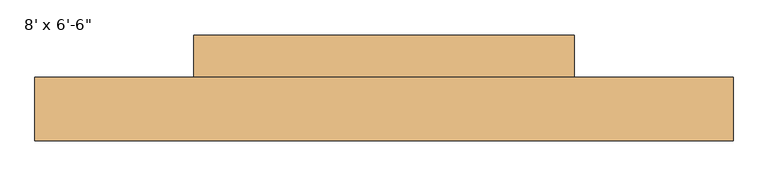
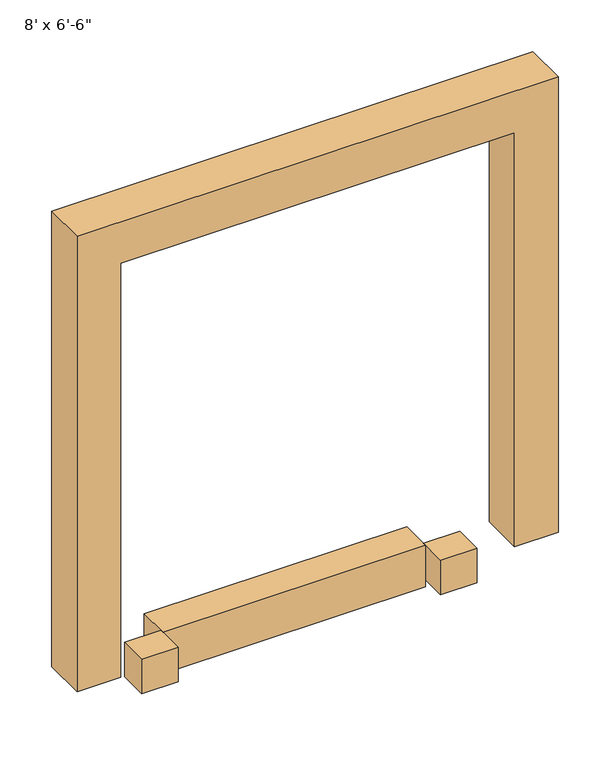
"""IFC4 building model written with IfcOpenShell, lengths in millimetres: door geometry."""

import ifcopenshell
import ifcopenshell.guid

model = None  # the IFC model being written
_history = None  # IfcOwnerHistory: only IFC2X3 demands one
_inside = {}  # id of a spatial element -> (the spatial element, [elements in it])
_under = {}  # id of a project, library or spatial element -> (it, [spatial elements below it])
_declared = {}  # id of a project -> (the project, [libraries it declares])
_typed = {}  # id of a type object -> (the type object, [elements of that type])
_made_of = {}  # id of a material, layer set ... -> (it, [elements and type objects made of it])


def new_model(schema):
    """Start an empty IFC model of exactly this schema.

    Asked for "IFC4X3", IfcOpenShell would pick the latest addendum, in which some entities
    have other attributes; the version numbers below select the first issue.
    IFC2X3 requires an IfcOwnerHistory on every rooted entity: one is made here for all.
    """
    global model, _history
    if schema == "IFC4X3":
        model = ifcopenshell.file(schema_version=(4, 3, 0, 0))
    else:
        model = ifcopenshell.file(schema=schema)
    _inside.clear()
    _under.clear()
    _declared.clear()
    _typed.clear()
    _made_of.clear()
    _history = None
    if model.schema == "IFC2X3":
        org = make("IfcOrganization", Name="unknown")
        user = make(
            "IfcPersonAndOrganization",
            ThePerson=make("IfcPerson", FamilyName="unknown"),
            TheOrganization=org,
        )
        app = make(
            "IfcApplication",
            ApplicationDeveloper=org,
            Version="unknown",
            ApplicationFullName="unknown",
            ApplicationIdentifier="unknown",
        )
        _history = make(
            "IfcOwnerHistory",
            OwningUser=user,
            OwningApplication=app,
            ChangeAction="ADDED",
            CreationDate=0,
        )
    return model


def make(cls, **values):
    """One entity of the class cls with the attributes given. An attribute that is None is left unset."""
    return model.create_entity(
        cls, **{name: value for name, value in values.items() if value is not None}
    )


def rooted(cls, **values):
    """An entity with a GlobalId (a new one), such as an element, a storey or a relation."""
    return make(cls, GlobalId=ifcopenshell.guid.new(), OwnerHistory=_history, **values)


def si_unit(unit_type, name, prefix=None):
    """IfcSIUnit, for example si_unit("LENGTHUNIT", "METRE", prefix="MILLI")."""
    return make("IfcSIUnit", UnitType=unit_type, Prefix=prefix, Name=name)


def assignment(units):
    """IfcUnitAssignment: the units of a project."""
    return None if units is None else make("IfcUnitAssignment", Units=units)


def point(xyz):
    """IfcCartesianPoint."""
    return None if xyz is None else make("IfcCartesianPoint", Coordinates=xyz)


def direction(xyz):
    """IfcDirection."""
    return None if xyz is None else make("IfcDirection", DirectionRatios=xyz)


def frame(location, z_axis=None, x_axis=None):
    """IfcAxis2Placement3D, a coordinate frame: its origin and axes. An axis left out is left unset."""
    return make(
        "IfcAxis2Placement3D",
        Location=point(location),
        Axis=direction(z_axis),
        RefDirection=direction(x_axis),
    )


def origin():
    """The frame at (0, 0, 0) with its axes left unset."""
    return frame((0.0, 0.0, 0.0))


def place(relative_to, where):
    """IfcLocalPlacement: puts the frame where relative to a parent placement (None: the world)."""
    return make(
        "IfcLocalPlacement", PlacementRelTo=relative_to, RelativePlacement=where
    )


def context(
    kind, dimensions, precision=None, world=None, true_north=None, identifier=None
):
    """IfcGeometricRepresentationContext, for example the 3D "Model" context."""
    return make(
        "IfcGeometricRepresentationContext",
        ContextIdentifier=identifier,
        ContextType=kind,
        CoordinateSpaceDimension=dimensions,
        Precision=precision,
        WorldCoordinateSystem=world,
        TrueNorth=true_north,
    )


def project(units=None, contexts=None):
    """IfcProject with its units and contexts."""
    return rooted(
        "IfcProject",
        Name="project",
        RepresentationContexts=contexts,
        UnitsInContext=assignment(units),
    )


def spatial(cls, under=None, at=None, **own):
    """A site, building, storey or space (cls), placed at a placement, below another one or the project."""
    s = rooted(cls, ObjectPlacement=at, **own)
    if under is not None:
        _under.setdefault(under.id(), (under, []))[1].append(s)
    return s


def polyline(points):
    """IfcPolyline through the points."""
    return make("IfcPolyline", Points=[point(p) for p in points])


def outline(outer, holes=None, kind="AREA"):
    """IfcArbitraryClosedProfileDef: a profile drawn as a closed curve; with holes, ...WithVoids."""
    if holes is None:
        return make("IfcArbitraryClosedProfileDef", ProfileType=kind, OuterCurve=outer)
    return make(
        "IfcArbitraryProfileDefWithVoids",
        ProfileType=kind,
        OuterCurve=outer,
        InnerCurves=holes,
    )


def extrude(swept, where, along, depth):
    """IfcExtrudedAreaSolid: the profile swept, set in the frame where, extruded along a direction by depth."""
    return make(
        "IfcExtrudedAreaSolid",
        SweptArea=swept,
        Position=where,
        ExtrudedDirection=direction(along),
        Depth=depth,
    )


def shape(context_of_items, identifier, shape_type, items):
    """IfcShapeRepresentation: the items that make up one representation, for example the "Body"."""
    return make(
        "IfcShapeRepresentation",
        ContextOfItems=context_of_items,
        RepresentationIdentifier=identifier,
        RepresentationType=shape_type,
        Items=items,
    )


def source(mapping_origin, context_of_items, identifier, shape_type, items):
    """IfcRepresentationMap: a shape defined once, which mapped items show again and again."""
    return make(
        "IfcRepresentationMap",
        MappingOrigin=mapping_origin,
        MappedRepresentation=shape(context_of_items, identifier, shape_type, items),
    )


def transform(
    local_origin,
    x_axis=None,
    y_axis=None,
    z_axis=None,
    scale=None,
    scale2=None,
    scale3=None,
    uniform=True,
):
    """IfcCartesianTransformationOperator3D, or its non-uniform kind. x_axis, y_axis, z_axis: its Axis1, 2, 3."""
    if uniform:
        return make(
            "IfcCartesianTransformationOperator3D",
            Axis1=direction(x_axis),
            Axis2=direction(y_axis),
            LocalOrigin=point(local_origin),
            Scale=scale,
            Axis3=direction(z_axis),
        )
    return make(
        "IfcCartesianTransformationOperator3DnonUniform",
        Axis1=direction(x_axis),
        Axis2=direction(y_axis),
        LocalOrigin=point(local_origin),
        Scale=scale,
        Axis3=direction(z_axis),
        Scale2=scale2,
        Scale3=scale3,
    )


def mapped(mapping_source, mapping_target):
    """IfcMappedItem: shows the shape of a source again, moved by a transform."""
    return make(
        "IfcMappedItem", MappingSource=mapping_source, MappingTarget=mapping_target
    )


def made_of(thing, what):
    """Note that an element or type object is made of a material, layer set ...; save() writes the relation."""
    if what is not None:
        _made_of.setdefault(what.id(), (what, []))[1].append(thing)
    return thing


def element(
    cls,
    number,
    at=None,
    inside=None,
    cuts=None,
    type_object=None,
    material=None,
    context=None,
    identifier="Body",
    shape_type=None,
    held_by="IfcProductDefinitionShape",
    body=None,
    shapes=None,
    **own,
):
    """One element of the class cls, such as IfcWall. Its Tag is "e" and its number.

    at: its placement. inside: the storey or other place that contains it. cuts: it is an
    opening in that element (IfcRelVoidsElement). A single representation is given by context,
    identifier, shape_type and body (its items); several are given by shapes. held_by: the class
    of the entity that holds the representations. save() writes the other relations.
    """
    e = rooted(cls, Tag="e%d" % number, ObjectPlacement=at, **own)
    if body is not None:
        shapes = [shape(context, identifier, shape_type, body)]
    if shapes is not None:
        e.Representation = make(held_by, Representations=shapes)
    if inside is not None:
        _inside.setdefault(inside.id(), (inside, []))[1].append(e)
    if cuts is not None:
        rooted(
            "IfcRelVoidsElement", RelatingBuildingElement=cuts, RelatedOpeningElement=e
        )
    if type_object is not None:
        _typed.setdefault(type_object.id(), (type_object, []))[1].append(e)
    return made_of(e, material)


def aggregate(whole, parts):
    """IfcRelAggregates: a whole, such as a stair, and the parts it consists of."""
    return rooted("IfcRelAggregates", RelatingObject=whole, RelatedObjects=parts)


def save(model, path):
    """Write the relations noted so far, then the file.

    IfcRelAggregates (storeys below a building ...), IfcRelContainedInSpatialStructure (elements
    in a storey), IfcRelDefinesByType, IfcRelAssociatesMaterial and IfcRelDeclares: one each for
    every whole, place, type object, material and project.
    """
    for whole, parts in _under.values():
        aggregate(whole, parts)
    for where, things in _inside.values():
        rooted(
            "IfcRelContainedInSpatialStructure",
            RelatedElements=things,
            RelatingStructure=where,
        )
    for kind, things in _typed.values():
        rooted("IfcRelDefinesByType", RelatedObjects=things, RelatingType=kind)
    for what, things in _made_of.values():
        rooted("IfcRelAssociatesMaterial", RelatedObjects=things, RelatingMaterial=what)
    for by, libraries in _declared.values():
        rooted("IfcRelDeclares", RelatingContext=by, RelatedDefinitions=libraries)
    model.write(path)


def door_9096417d(model_context):
    return source(origin(), model_context, "Body", "SweptSolid", [
        extrude(outline(polyline([(0.0, 1676.4), (3352.8, 1676.4), (3352.8, -1676.4), (0.0, -1676.4), (0.0, -1371.6), (3048.0, -1371.6), (3048.0, 1371.6), (0.0, 1371.6), (0.0, 1676.4)])), frame((0.0, -331.7875, 0.0), z_axis=(0.0, 1.0, 0.0), x_axis=(0.0, 0.0, 1.0)), (0.0, 0.0, 1.0), 304.8),
        extrude(outline(polyline([(-1168.4, -230.1875), (-1168.4, -26.9875), (-914.4, -26.9875), (-914.4, -230.1875), (-1168.4, -230.1875)])), frame((0.0, 0.0, -254.0), z_axis=(0.0, 0.0, 1.0), x_axis=(1.0, 0.0, 0.0)), (0.0, 0.0, 1.0), 254.0),
        extrude(outline(polyline([(914.4, -230.1875), (914.4, -26.9875), (1168.4, -26.9875), (1168.4, -230.1875), (914.4, -230.1875)])), frame((0.0, 0.0, -254.0), z_axis=(0.0, 0.0, 1.0), x_axis=(1.0, 0.0, 0.0)), (0.0, 0.0, 1.0), 254.0),
        extrude(outline(polyline([(-914.4, -52.3875), (-914.4, 176.2125), (914.4, 176.2125), (914.4, -52.3875), (-914.4, -52.3875)])), frame((0.0, 0.0, -304.8), z_axis=(0.0, 0.0, 1.0), x_axis=(1.0, 0.0, 0.0)), (0.0, 0.0, 1.0), 304.8),
    ])


if __name__ == "__main__":
    model = new_model("IFC4")
    model_context = context("Model", 3, world=origin())
    ifc_project = project(units=[si_unit("LENGTHUNIT", "METRE", prefix="MILLI")], contexts=[model_context])
    site = spatial("IfcSite", under=ifc_project)
    building = spatial("IfcBuilding", under=site)
    placement = place(None, origin())
    door_shape = door_9096417d(model_context)
    element("IfcDoor", 1, ObjectType="OHD_WPADS_2491 : 8' x 6'-6\"", at=placement, inside=building, context=model_context, shape_type="MappedRepresentation", body=[
        mapped(door_shape, transform((0.0, 0.0, 0.0), x_axis=(1.0, 0.0, 0.0), y_axis=(0.0, 1.0, 0.0), z_axis=(0.0, 0.0, 1.0))),
    ])
    save(model, "model.ifc")

# Revit data of these elements
# Type "OHD_WPADS_2491 : 8' x 6'-6\""
#   Type Mark = "22"
#   Assembly Code = "B2030410"
#   Height = 1981.2 mm
#   Thickness = 38.1 mm
#   Width = 2438.4 mm
#   Define Thermal Properties by = 0
#   Material = none
#   Function = (empty or 0)
#   Wall Closure = (empty or 0)
# Element 1 (IfcDoor, "OHD_WPADS_2491 : 8' x 6'-6\"")
#   Materials on its faces: "BUMPER", "PAD", "LEVELER"
# Materials
#   "BUMPER": class "Unassigned", colour RGB 63 63 63, transparency 0, Comments = "Rendering appearance not upgraded ", Cost = 0
#   "PAD": class "Unassigned", colour RGB 255 255 0, transparency 0, Comments = "Rendering appearance not upgraded ", Cost = 0
#   "LEVELER": class "Unassigned", colour RGB 189 187 185, transparency 0, Comments = "Rendering appearance not upgraded ", Cost = 0
